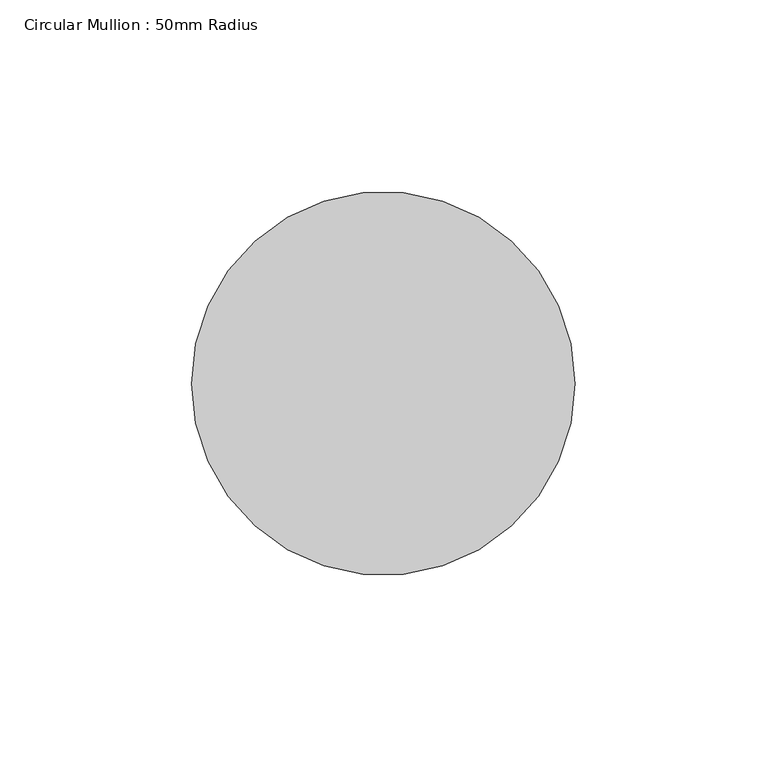
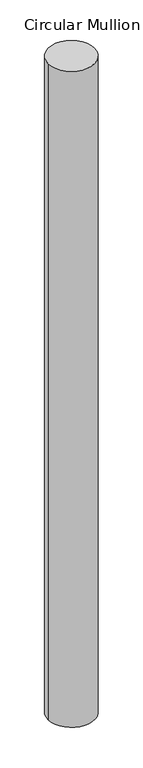
"""IFC4 building model written with IfcOpenShell, lengths in millimetres: member geometry, Circular Mullion : 50mm Radius."""

from ifc_helpers import new_model, si_unit, point, frame, origin, origin_2d, place, context, project, spatial, circle_curve, trimmed, segment, composite_curve, outline, extrude, source, transform, mapped, element, save


def circular_mullion_50mm_radius_812a657b(model_context):
    return source(origin(), model_context, "Body", "SweptSolid", [
        extrude(outline(composite_curve([segment(trimmed(circle_curve(origin_2d(), 50.0), [point((50.0, 0.0))], [point((-50.0, 0.0))], False, "CARTESIAN"), True, "CONTINUOUS"), segment(trimmed(circle_curve(origin_2d(), 50.0), [point((-50.0, 0.0))], [point((50.0, 0.0))], False, "CARTESIAN"), True, "CONTINUOUS")], self_intersect=False)), frame((0.0, 0.0, -1490.3797869), z_axis=(0.0, 0.0, 1.0), x_axis=(1.0, 0.0, 0.0)), (0.0, 0.0, 1.0), 1490.3797869),
    ])


if __name__ == "__main__":
    model = new_model("IFC4")
    model_context = context("Model", 3, world=origin())
    ifc_project = project(units=[si_unit("LENGTHUNIT", "METRE", prefix="MILLI")], contexts=[model_context])
    site = spatial("IfcSite", under=ifc_project)
    building = spatial("IfcBuilding", under=site)
    placement = place(None, origin())
    circular_mullion_50mm_radius_shape = circular_mullion_50mm_radius_812a657b(model_context)
    element("IfcMember", 1, ObjectType="Circular Mullion : 50mm Radius", at=placement, inside=building, context=model_context, shape_type="MappedRepresentation", body=[
        mapped(circular_mullion_50mm_radius_shape, transform((0.0, 0.0, 0.0), x_axis=(1.0, 0.0, 0.0), y_axis=(0.0, 1.0, 0.0), z_axis=(0.0, 0.0, 1.0))),
    ])
    save(model, "model.ifc")

# Revit data of these elements
# Type "Circular Mullion : 50mm Radius"
#   built-in parameter 1007350 = 0.164042 (stored number, unit not read)
# Element 1 (IfcMember, "Circular Mullion : 50mm Radius")
#   Materials on its faces: "Aluminium"
# Materials
#   "Aluminium": class "Metal", colour RGB 247 247 247, transparency 0, Description = "Aluminium 6061", Cost = 0
